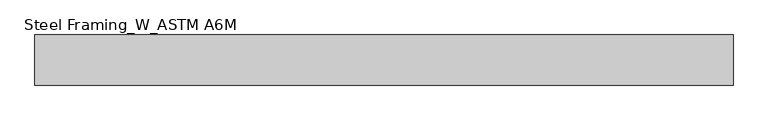
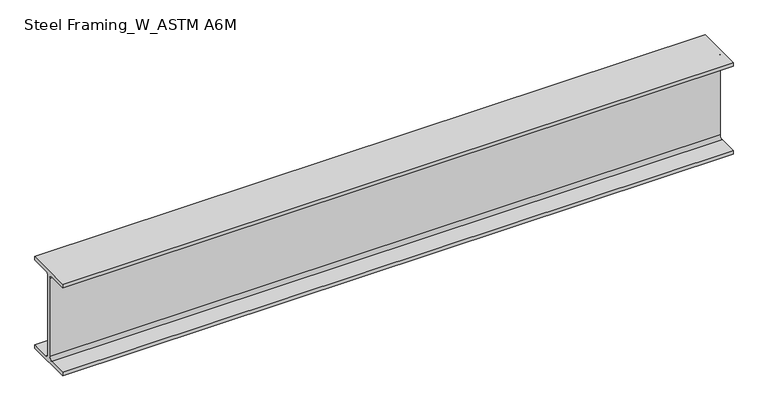
"""IFC4 building model written with IfcOpenShell, lengths in millimetres: beam geometry, Steel Framing_W_ASTM A6M : H_SB_AR_S02_W200x22.5_B7."""

from ifc_helpers import new_model, si_unit, point, frame, frame_2d, origin, place, context, project, spatial, polyline, circle_curve, trimmed, segment, composite_curve, outline, extrude, source, transform, mapped, element, save


def steel_framing_w_astm_a6m_b276909d(model_context):
    return source(origin(), model_context, "Body", "SweptSolid", [
        extrude(outline(composite_curve([segment(polyline([(51.0, -95.0), (51.0, -103.0), (-51.0, -103.0), (-51.0, -95.0), (-10.71, -95.0)]), True, "CONTINUOUS"), segment(trimmed(circle_curve(frame_2d((-10.71, -87.4)), 7.6), [point((-10.71, -95.0))], [point((-3.11, -87.4))], True, "CARTESIAN"), True, "CONTINUOUS"), segment(polyline([(-3.11, -87.4), (-3.11, 87.4)]), True, "CONTINUOUS"), segment(trimmed(circle_curve(frame_2d((-10.71, 87.4)), 7.6), [point((-3.11, 87.4))], [point((-10.71, 95.0))], True, "CARTESIAN"), True, "CONTINUOUS"), segment(polyline([(-10.71, 95.0), (-51.0, 95.0), (-51.0, 103.0), (51.0, 103.0), (51.0, 95.0), (10.71, 95.0)]), True, "CONTINUOUS"), segment(trimmed(circle_curve(frame_2d((10.71, 87.4)), 7.6), [point((10.71, 95.0))], [point((3.11, 87.4))], True, "CARTESIAN"), True, "CONTINUOUS"), segment(polyline([(3.11, 87.4), (3.11, -87.4)]), True, "CONTINUOUS"), segment(trimmed(circle_curve(frame_2d((10.71, -87.4)), 7.6), [point((3.11, -87.4))], [point((10.71, -95.0))], True, "CARTESIAN"), True, "CONTINUOUS"), segment(polyline([(10.71, -95.0), (51.0, -95.0)]), True, "CONTINUOUS")], self_intersect=False)), frame((-710.3, 0.0, 0.0), z_axis=(1.0, 0.0, 0.0), x_axis=(0.0, 1.0, 0.0)), (0.0, 0.0, 1.0), 1420.6),
    ])


if __name__ == "__main__":
    model = new_model("IFC4")
    model_context = context("Model", 3, world=origin())
    ifc_project = project(units=[si_unit("LENGTHUNIT", "METRE", prefix="MILLI")], contexts=[model_context])
    site = spatial("IfcSite", under=ifc_project)
    building = spatial("IfcBuilding", under=site)
    placement = place(None, origin())
    steel_framing_w_astm_a6m_shape = steel_framing_w_astm_a6m_b276909d(model_context)
    element("IfcBeam", 1, ObjectType="Steel Framing_W_ASTM A6M : H_SB_AR_S02_W200x22.5_B7", at=placement, inside=building, context=model_context, shape_type="MappedRepresentation", body=[
        mapped(steel_framing_w_astm_a6m_shape, transform((0.0, 0.0, 0.0), x_axis=(1.0, 0.0, 0.0), y_axis=(0.0, 1.0, 0.0), z_axis=(0.0, 0.0, 1.0))),
    ])
    save(model, "model.ifc")

# Revit data of these elements
# Type "Steel Framing_W_ASTM A6M : H_SB_AR_S02_W200x22.5_B7"
#   Type Mark = "B7"
#   Section Name Key = "W8x15"
#   Width = 10.2 cm
#   Web Thickness = 0.622 cm
#   Web Fillet = 0.76 cm
#   Warping Constant = 13900.0 cm⁶
#   Torsional Moment of Inertia = 5.70 cm⁴
#   Section Area = 28.6 cm²
#   Plastic Modulus weak axis = 43.8 cm³
#   Plastic Modulus strong axis = 223.0 cm³
#   Perimeter = 0.795 m²/m
#   Nominal Weight = 22.50 kgf/m
#   Moment of Inertia weak axis = 142.00 cm⁴
#   Moment of Inertia strong axis = 2000.00 cm⁴
#   Height = 20.6 cm
#   Flange Thickness = 0.8 cm
#   Elastic Modulus weak axis = 27.9 cm³
#   Elastic Modulus strong axis = 193.0 cm³
#   Centroid Vertical = 10.3 cm
#   Centroid Horizontal = 5.1 cm
#   Length [instance default] = 1500 mm
#   Structural Material [instance default] = Steel, 45-345
#   Bolt Spacing = 0
#   Assembly Code = ""
# Element 1 (IfcBeam, "Steel Framing_W_ASTM A6M : H_SB_AR_S02_W200x22.5_B7")
#   Materials on its faces: "Steel, 45-345"
# Materials
#   "Steel, 45-345": class "Metal", colour RGB 189 187 185, transparency 0, Description = "Steel 345 MPa", Cost = 0
